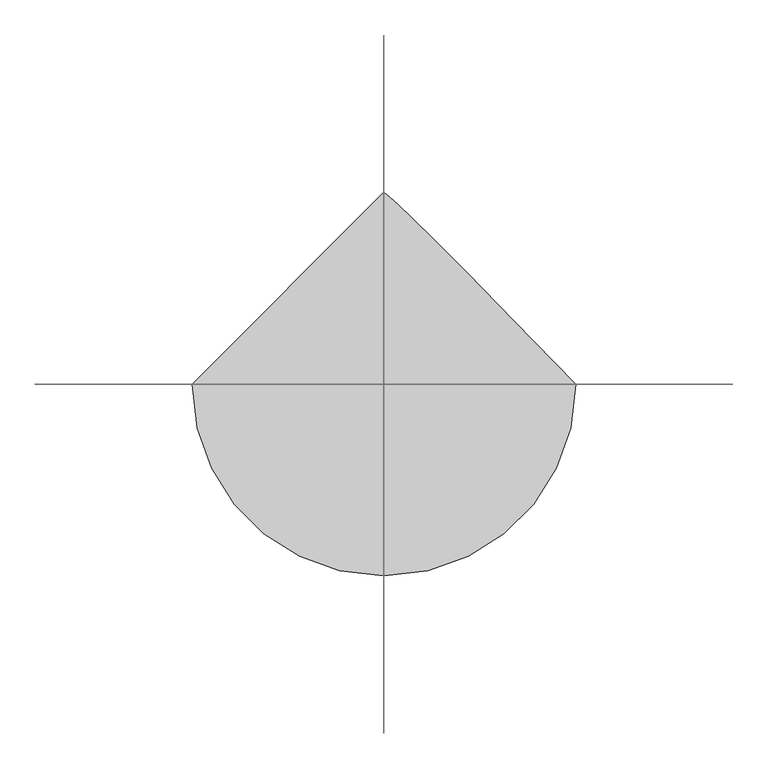
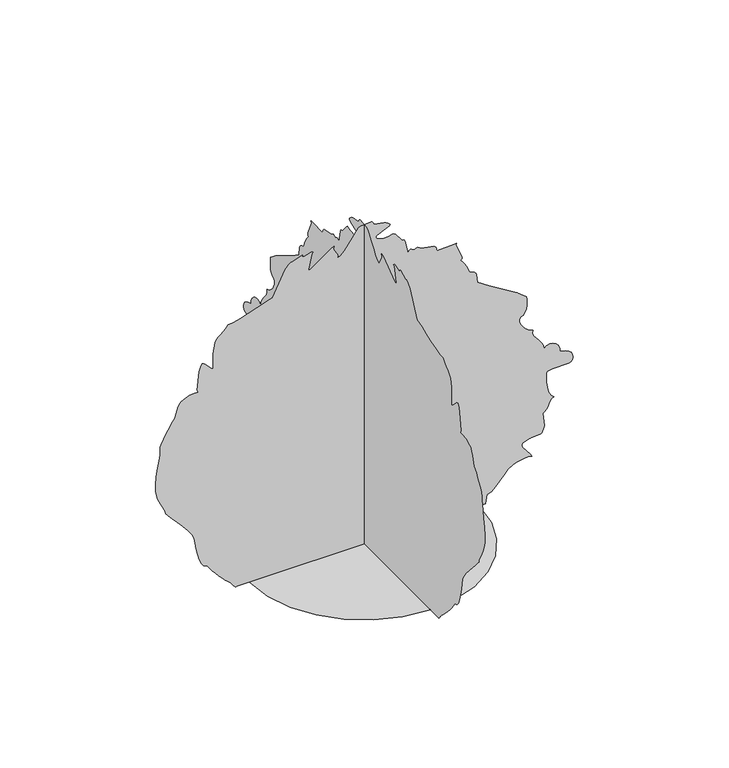
"""IFC4 building model written with IfcOpenShell, lengths in millimetres: proxy geometry, vibernum 26767 : vibernum 26767."""

import ifcopenshell
import ifcopenshell.guid

model = None  # the IFC model being written
_history = None  # IfcOwnerHistory: only IFC2X3 demands one
_inside = {}  # id of a spatial element -> (the spatial element, [elements in it])
_under = {}  # id of a project, library or spatial element -> (it, [spatial elements below it])
_declared = {}  # id of a project -> (the project, [libraries it declares])
_typed = {}  # id of a type object -> (the type object, [elements of that type])
_made_of = {}  # id of a material, layer set ... -> (it, [elements and type objects made of it])


def new_model(schema):
    """Start an empty IFC model of exactly this schema.

    Asked for "IFC4X3", IfcOpenShell would pick the latest addendum, in which some entities
    have other attributes; the version numbers below select the first issue.
    IFC2X3 requires an IfcOwnerHistory on every rooted entity: one is made here for all.
    """
    global model, _history
    if schema == "IFC4X3":
        model = ifcopenshell.file(schema_version=(4, 3, 0, 0))
    else:
        model = ifcopenshell.file(schema=schema)
    _inside.clear()
    _under.clear()
    _declared.clear()
    _typed.clear()
    _made_of.clear()
    _history = None
    if model.schema == "IFC2X3":
        org = make("IfcOrganization", Name="unknown")
        user = make(
            "IfcPersonAndOrganization",
            ThePerson=make("IfcPerson", FamilyName="unknown"),
            TheOrganization=org,
        )
        app = make(
            "IfcApplication",
            ApplicationDeveloper=org,
            Version="unknown",
            ApplicationFullName="unknown",
            ApplicationIdentifier="unknown",
        )
        _history = make(
            "IfcOwnerHistory",
            OwningUser=user,
            OwningApplication=app,
            ChangeAction="ADDED",
            CreationDate=0,
        )
    return model


def make(cls, **values):
    """One entity of the class cls with the attributes given. An attribute that is None is left unset."""
    return model.create_entity(
        cls, **{name: value for name, value in values.items() if value is not None}
    )


def rooted(cls, **values):
    """An entity with a GlobalId (a new one), such as an element, a storey or a relation."""
    return make(cls, GlobalId=ifcopenshell.guid.new(), OwnerHistory=_history, **values)


def si_unit(unit_type, name, prefix=None):
    """IfcSIUnit, for example si_unit("LENGTHUNIT", "METRE", prefix="MILLI")."""
    return make("IfcSIUnit", UnitType=unit_type, Prefix=prefix, Name=name)


def assignment(units):
    """IfcUnitAssignment: the units of a project."""
    return None if units is None else make("IfcUnitAssignment", Units=units)


def point(xyz):
    """IfcCartesianPoint."""
    return None if xyz is None else make("IfcCartesianPoint", Coordinates=xyz)


def direction(xyz):
    """IfcDirection."""
    return None if xyz is None else make("IfcDirection", DirectionRatios=xyz)


def frame(location, z_axis=None, x_axis=None):
    """IfcAxis2Placement3D, a coordinate frame: its origin and axes. An axis left out is left unset."""
    return make(
        "IfcAxis2Placement3D",
        Location=point(location),
        Axis=direction(z_axis),
        RefDirection=direction(x_axis),
    )


def origin():
    """The frame at (0, 0, 0) with its axes left unset."""
    return frame((0.0, 0.0, 0.0))


def place(relative_to, where):
    """IfcLocalPlacement: puts the frame where relative to a parent placement (None: the world)."""
    return make(
        "IfcLocalPlacement", PlacementRelTo=relative_to, RelativePlacement=where
    )


def context(
    kind, dimensions, precision=None, world=None, true_north=None, identifier=None
):
    """IfcGeometricRepresentationContext, for example the 3D "Model" context."""
    return make(
        "IfcGeometricRepresentationContext",
        ContextIdentifier=identifier,
        ContextType=kind,
        CoordinateSpaceDimension=dimensions,
        Precision=precision,
        WorldCoordinateSystem=world,
        TrueNorth=true_north,
    )


def project(units=None, contexts=None):
    """IfcProject with its units and contexts."""
    return rooted(
        "IfcProject",
        Name="project",
        RepresentationContexts=contexts,
        UnitsInContext=assignment(units),
    )


def spatial(cls, under=None, at=None, **own):
    """A site, building, storey or space (cls), placed at a placement, below another one or the project."""
    s = rooted(cls, ObjectPlacement=at, **own)
    if under is not None:
        _under.setdefault(under.id(), (under, []))[1].append(s)
    return s


def point_list(points):
    """IfcCartesianPointList2D or 3D."""
    cls = (
        "IfcCartesianPointList2D" if len(points[0]) == 2 else "IfcCartesianPointList3D"
    )
    return make(cls, CoordList=points)


def triangles(points, corners, closed=None, point_numbers=None):
    """IfcTriangulatedFaceSet: each triangle names its three corners, points numbered from 1."""
    return make(
        "IfcTriangulatedFaceSet",
        Coordinates=point_list(points),
        Closed=closed,
        CoordIndex=corners,
        PnIndex=point_numbers,
    )


def shape(context_of_items, identifier, shape_type, items):
    """IfcShapeRepresentation: the items that make up one representation, for example the "Body"."""
    return make(
        "IfcShapeRepresentation",
        ContextOfItems=context_of_items,
        RepresentationIdentifier=identifier,
        RepresentationType=shape_type,
        Items=items,
    )


def source(mapping_origin, context_of_items, identifier, shape_type, items):
    """IfcRepresentationMap: a shape defined once, which mapped items show again and again."""
    return make(
        "IfcRepresentationMap",
        MappingOrigin=mapping_origin,
        MappedRepresentation=shape(context_of_items, identifier, shape_type, items),
    )


def transform(
    local_origin,
    x_axis=None,
    y_axis=None,
    z_axis=None,
    scale=None,
    scale2=None,
    scale3=None,
    uniform=True,
):
    """IfcCartesianTransformationOperator3D, or its non-uniform kind. x_axis, y_axis, z_axis: its Axis1, 2, 3."""
    if uniform:
        return make(
            "IfcCartesianTransformationOperator3D",
            Axis1=direction(x_axis),
            Axis2=direction(y_axis),
            LocalOrigin=point(local_origin),
            Scale=scale,
            Axis3=direction(z_axis),
        )
    return make(
        "IfcCartesianTransformationOperator3DnonUniform",
        Axis1=direction(x_axis),
        Axis2=direction(y_axis),
        LocalOrigin=point(local_origin),
        Scale=scale,
        Axis3=direction(z_axis),
        Scale2=scale2,
        Scale3=scale3,
    )


def mapped(mapping_source, mapping_target):
    """IfcMappedItem: shows the shape of a source again, moved by a transform."""
    return make(
        "IfcMappedItem", MappingSource=mapping_source, MappingTarget=mapping_target
    )


def made_of(thing, what):
    """Note that an element or type object is made of a material, layer set ...; save() writes the relation."""
    if what is not None:
        _made_of.setdefault(what.id(), (what, []))[1].append(thing)
    return thing


def element(
    cls,
    number,
    at=None,
    inside=None,
    cuts=None,
    type_object=None,
    material=None,
    context=None,
    identifier="Body",
    shape_type=None,
    held_by="IfcProductDefinitionShape",
    body=None,
    shapes=None,
    **own,
):
    """One element of the class cls, such as IfcWall. Its Tag is "e" and its number.

    at: its placement. inside: the storey or other place that contains it. cuts: it is an
    opening in that element (IfcRelVoidsElement). A single representation is given by context,
    identifier, shape_type and body (its items); several are given by shapes. held_by: the class
    of the entity that holds the representations. save() writes the other relations.
    """
    e = rooted(cls, Tag="e%d" % number, ObjectPlacement=at, **own)
    if body is not None:
        shapes = [shape(context, identifier, shape_type, body)]
    if shapes is not None:
        e.Representation = make(held_by, Representations=shapes)
    if inside is not None:
        _inside.setdefault(inside.id(), (inside, []))[1].append(e)
    if cuts is not None:
        rooted(
            "IfcRelVoidsElement", RelatingBuildingElement=cuts, RelatedOpeningElement=e
        )
    if type_object is not None:
        _typed.setdefault(type_object.id(), (type_object, []))[1].append(e)
    return made_of(e, material)


def aggregate(whole, parts):
    """IfcRelAggregates: a whole, such as a stair, and the parts it consists of."""
    return rooted("IfcRelAggregates", RelatingObject=whole, RelatedObjects=parts)


def save(model, path):
    """Write the relations noted so far, then the file.

    IfcRelAggregates (storeys below a building ...), IfcRelContainedInSpatialStructure (elements
    in a storey), IfcRelDefinesByType, IfcRelAssociatesMaterial and IfcRelDeclares: one each for
    every whole, place, type object, material and project.
    """
    for whole, parts in _under.values():
        aggregate(whole, parts)
    for where, things in _inside.values():
        rooted(
            "IfcRelContainedInSpatialStructure",
            RelatedElements=things,
            RelatingStructure=where,
        )
    for kind, things in _typed.values():
        rooted("IfcRelDefinesByType", RelatedObjects=things, RelatingType=kind)
    for what, things in _made_of.values():
        rooted("IfcRelAssociatesMaterial", RelatedObjects=things, RelatingMaterial=what)
    for by, libraries in _declared.values():
        rooted("IfcRelDeclares", RelatingContext=by, RelatedDefinitions=libraries)
    model.write(path)


def entourage_5c4a15e9(model_context):
    return source(origin(), model_context, "Body", "Tessellation", [
        triangles([(-310.4009663, 0.0, 0.0), (-302.1967432, -71.1236111, 0.0), (-278.8261857, -136.4392555, 0.0), (-242.1615087, -194.0757083, 0.0), (-194.0757083, -242.1615087, 0.0), (-136.4392555, -278.8261857, 0.0), (-71.1236111, -302.1967432, 0.0), (1.36e-05, -310.4009663, 0.0), (71.1236111, -302.1967432, 0.0), (136.4392555, -278.8261857, 0.0), (194.0757083, -242.1615087, 0.0), (242.1615087, -194.0757083, 0.0), (278.8261857, -136.4392555, 0.0), (302.1967432, -71.1236111, 0.0), (310.4009663, 2.71e-05, 0.0), (209.5283262, 103.4718092, 0.0), (134.7455816, 179.6535872, 0.0), (81.7052599, 233.0934394, 0.0), (46.0591254, 268.3410517, 0.0), (23.45852, 289.9412231, 0.0), (9.5549798, 302.4456561, 0.0), (-4.07e-05, 310.4009663, 0.0), (-352.7554667, 2.15e-05, 4.3495503), (-355.9965117, 2.13e-05, 8.4826161), (-359.0826241, 2.1e-05, 12.3234041), (-362.0188548, 2.08e-05, 15.7959676), (-364.8077834, 2.07e-05, 18.8245652), (-367.457004, 2.05e-05, 21.3332227), (-369.9665528, 2.04e-05, 23.2460988), (-375.8161594, 2.01e-05, 28.5320975), (-383.5606359, 1.96e-05, 36.3306653), (-392.4582396, 1.9e-05, 45.9079945), (-401.7775108, 1.84e-05, 56.5300297), (-410.7742001, 1.78e-05, 67.463215), (-418.7091808, 1.71e-05, 77.9737471), (-424.8483773, 1.66e-05, 87.3278091), (-434.3200376, 1.64e-05, 90.3102761), (-441.518399, 1.59e-05, 99.1873323), (-446.9133459, 1.51e-05, 112.4136326), (-450.9672046, 1.41e-05, 128.4448579), (-454.1523663, 1.31e-05, 145.7354086), (-456.9311211, 1.21e-05, 162.7404662), (-459.7733894, 1.12e-05, 177.9152122), (-465.8821009, 1.05e-05, 189.8085088), (-476.9463238, 9.6e-06, 205.0848474), (-490.9620744, 8.5e-06, 222.0754346), (-505.927767, 7.5e-06, 239.1112225), (-519.8393452, 6.6e-06, 254.5234358), (-530.6927888, 5.9e-06, 266.6443348), (-536.4840051, 5.5e-06, 273.804599), (-537.980062, 5.1e-06, 279.9056801), (-541.2769901, 4.6e-06, 287.7695352), (-545.6533945, 4.1e-06, 296.6874683), (-550.3904963, 3.6e-06, 305.9584685), (-554.7669371, 3e-06, 314.8764198), (-558.0638288, 2.6e-06, 322.7377496), (-559.5599221, 2.2e-06, 328.8413741), (-564.0633173, 1.1e-06, 346.2505222), (-564.6424607, -1e-07, 367.0963428), (-562.5393188, -1.4e-06, 389.5906094), (-558.9909525, -2.8e-06, 411.9375375), (-555.2393646, -4e-06, 432.3439227), (-552.5215799, -5e-06, 449.0164879), (-552.0770576, -5.6e-06, 460.1619922), (-551.4522048, -6.2e-06, 469.7809908), (-548.1832546, -6.8e-06, 479.8495623), (-543.0422894, -7.4e-06, 490.1772022), (-536.8090942, -8.1e-06, 500.5785295), (-530.2609838, -8.7e-06, 510.8553732), (-524.1776705, -9.2e-06, 520.822352), (-519.3338891, -9.8e-06, 530.2863819), (-514.6958364, -1.01e-05, 534.5764544), (-511.1779552, -1.05e-05, 541.7037083), (-508.3280565, -1.1e-05, 550.5352913), (-505.7042341, -1.16e-05, 559.930757), (-502.8569152, -1.21e-05, 568.7597966), (-499.3364542, -1.25e-05, 575.8870505), (-494.6984015, -1.28e-05, 580.1796301), (-488.7141738, -1.3e-05, 583.3724221), (-483.0575787, -1.32e-05, 586.1308657), (-477.4467293, -1.33e-05, 588.3914835), (-471.5996298, -1.34e-05, 590.0856388), (-465.2318499, -1.35e-05, 591.1448401), (-458.0563431, -1.35e-05, 591.5029578), (-449.7962731, -1.35e-05, 591.0940438), (-452.0898831, -1.38e-05, 597.7844058), (-446.8498687, -1.69e-05, 648.1323137), (-442.8239516, -1.75e-05, 659.7223766), (-438.0639951, -1.8e-05, 668.1551468), (-434.5155925, -1.8e-05, 667.6064884), (-430.9748566, -1.79e-05, 665.0360058), (-414.5257879, -1.68e-05, 647.428723), (-409.2578319, -1.66e-05, 644.4162615), (-408.9962199, -1.74e-05, 657.4007887), (-409.1181238, -1.79e-05, 666.2653639), (-409.3213454, -1.83e-05, 672.7017443), (-409.3035413, -1.87e-05, 678.4040852), (-408.7625133, -1.91e-05, 685.0639257), (-407.3934834, -1.96e-05, 694.3755667), (-404.8915649, -2.04e-05, 708.0306198), (-403.2913719, -2.1e-05, 717.4769182), (-399.8064829, -2.14e-05, 724.3451036), (-394.8255369, -2.17e-05, 729.6460882), (-388.7295427, -2.2e-05, 734.3907841), (-381.9096102, -2.23e-05, 739.5952629), (-374.7468206, -2.27e-05, 746.2703642), (-367.6271971, -2.33e-05, 755.4296162), (-354.5182589, -2.33e-05, 756.2449734), (-335.3386883, -2.36e-05, 761.043009), (-312.9155657, -2.4e-05, 768.2718555), (-290.0885433, -2.45e-05, 776.3821163), (-269.6872632, -2.49e-05, 783.819235), (-254.5437653, -2.53e-05, 789.0313442), (-247.4939957, -2.53e-05, 790.4715179), (-213.6794536, -2.94e-05, 858.769602), (-205.2583288, -3e-05, 869.5493946), (-197.3670409, -3.03e-05, 874.0807314), (-193.2331907, -3.03e-05, 873.8495682), (-168.7295447, -3.09e-05, 884.1188541), (-166.460806, -3.09e-05, 883.4558859), (-168.0742249, -3.06e-05, 879.0896553), (-161.877383, -3.06e-05, 879.3893463), (-144.3734641, -3.09e-05, 884.8376329), (-141.0938133, -3.09e-05, 884.1543898), (-137.9627544, -3.07e-05, 881.4086271), (-140.7920603, -3.07e-05, 880.4332506), (-150.2901451, -2.82e-05, 838.0508085), (-150.4359393, -2.79e-05, 834.0097034), (-142.0369153, -2.81e-05, 837.3624784), (-89.9201382, -3.04e-05, 875.4065952), (-81.5211142, -3.06e-05, 878.7594429), (-83.236371, -3.02e-05, 872.9860308), (-82.0336828, -2.99e-05, 867.6621552), (-72.5891921, -2.9e-05, 852.5922901), (-71.3862495, -2.87e-05, 847.2684872), (-73.1015109, -2.84e-05, 841.495075), (-63.556186, -2.86e-05, 845.6047806), (-53.0855361, -2.92e-05, 856.2092932), (-42.3674857, -3.01e-05, 870.5983858), (-32.0797166, -3.1e-05, 886.0492596), (-22.9007347, -3.19e-05, 899.8541582), (-15.50783, -3.24e-05, 909.2952971), (-10.5790577, -3.25e-05, 911.6575075), (18.9106201, -3.27e-05, 914.4007267), (21.5322068, -3.27e-05, 913.1789989), (23.8564858, -3.25e-05, 909.8845779), (26.6850082, -3.21e-05, 903.8622711), (53.36646, -3.19e-05, 899.8287237), (58.7731068, -3.17e-05, 897.4639698), (63.9669031, -3.15e-05, 893.9232702), (69.0938976, -3.12e-05, 888.8939987), (68.0601171, -3.1e-05, 885.5234196), (63.3263127, -3.08e-05, 882.1706446), (34.7215748, -3.01e-05, 870.0904226), (31.9859905, -2.99e-05, 867.6900604), (32.133565, -2.97e-05, 863.7226427), (35.5686638, -2.95e-05, 860.1538925), (41.5277613, -2.93e-05, 857.2862623), (49.2473392, -2.92e-05, 855.4244574), (57.9630999, -2.92e-05, 854.8808859), (66.9122902, -2.92e-05, 855.9553116), (75.3308715, -2.94e-05, 858.9575993), (79.5358429, -2.94e-05, 858.9905914), (84.1909094, -2.92e-05, 855.1374109), (99.0570351, -2.8e-05, 835.8054514), (103.7123468, -2.78e-05, 831.9522709), (107.9173227, -2.78e-05, 831.9827196), (110.5566329, -2.75e-05, 826.9687815), (117.7400153, -2.54e-05, 791.6018269), (122.069702, -2.57e-05, 796.2169521), (125.2845857, -2.58e-05, 797.6521116), (127.9442162, -2.57e-05, 797.0729319), (133.8415943, -2.56e-05, 794.512623), (138.1999856, -2.56e-05, 794.8580961), (144.2457012, -2.58e-05, 797.8374928), (154.0983702, -2.54e-05, 791.6500797), (188.4892397, -2.5e-05, 784.7844378), (193.5639118, -2.47e-05, 779.5723286), (196.3218285, -2.41e-05, 769.7729994), (243.3426139, -2.42e-05, 771.0379658), (249.3334547, -2.43e-05, 772.2673239), (247.7520468, -2.39e-05, 766.8596598), (263.6852313, -2.17e-05, 729.0644377), (264.3888039, -2.13e-05, 722.3968941), (260.2486133, -2.11e-05, 719.5673429), (264.4396183, -2.09e-05, 715.6404751), (268.5899827, -2.05e-05, 710.080422), (272.58794, -2.02e-05, 703.4306826), (276.3268288, -1.97e-05, 696.2399878), (279.6948645, -1.93e-05, 689.0492203), (282.5828423, -1.89e-05, 682.4020243), (284.8815392, -1.86e-05, 676.8470581), (292.1535699, -1.84e-05, 674.5203833), (297.5205933, -1.82e-05, 671.6629269), (301.2772681, -1.8e-05, 668.0231054), (303.7181983, -1.78e-05, 663.3520243), (306.0880391, -1.64e-05, 640.6748474), (337.5484735, -1.51e-05, 619.285528), (412.8366832, -1.23e-05, 572.7882208), (438.1198783, -1.12e-05, 553.4791523), (439.8826341, -1.08e-05, 546.9589471), (439.9893136, -9.7e-06, 528.3128105), (438.1224217, -9.1e-06, 518.4956772), (434.833124, -8.6e-06, 509.8850836), (430.0172479, -8.2e-06, 503.634157), (423.57073, -8.1e-06, 500.8960247), (419.6083265, -7.7e-06, 495.2673712), (419.9613936, -7.3e-06, 487.2053996), (423.7561475, -6.7e-06, 477.8835849), (430.1112465, -6.1e-06, 468.4703513), (438.1503633, -5.6e-06, 460.136594), (446.9946273, -5.3e-06, 454.0533171), (455.7652765, -5.1e-06, 451.3913793), (454.5663671, -4.6e-06, 443.4767461), (457.9420332, -4.1e-06, 435.1353584), (464.2260246, -3.6e-06, 426.3952306), (471.7495116, -3.1e-06, 417.2791446), (478.8462805, -2.5e-06, 407.8151147), (483.8449943, -1.9e-06, 398.025923), (485.0794393, -1.3e-06, 387.9344968), (492.6181506, -1.7e-06, 394.3632468), (501.3405107, -1.8e-06, 396.5095548), (510.2914905, -1.8e-06, 394.9982735), (518.5109379, -1.5e-06, 390.4541831), (525.0463675, -1.1e-06, 383.5047526), (528.9401705, -5e-07, 374.7773057), (529.2322675, 0.0, 364.8966951), (543.28359, 2e-07, 361.6200783), (553.2505325, 5e-07, 356.9591709), (559.7300789, 8e-07, 351.3864369), (563.3267344, 1.2e-06, 345.3742312), (564.6424607, 1.5e-06, 339.3975975), (564.2741693, 1.9e-06, 333.9264562), (562.8263652, 2.1e-06, 329.438249), (558.5058077, 2.4e-06, 325.0237292), (551.6808246, 2.5e-06, 323.3371679), (508.3052018, 2.5e-06, 323.4667022), (495.6814084, 2.7e-06, 320.1113837), (493.0550426, 3e-06, 315.2853702), (491.9247336, 3.6e-06, 304.683401), (492.3870237, 4.5e-06, 290.5000371), (494.5434691, 5.4e-06, 274.934908), (498.4855614, 6.3e-06, 260.1850997), (504.3148567, 7e-06, 248.4462268), (512.1304407, 7.4e-06, 241.918682), (506.1944658, 7.6e-06, 237.9293542), (502.0110729, 7.9e-06, 232.375896), (498.8894248, 8.3e-06, 225.9143899), (496.1360682, 8.7e-06, 219.2011551), (493.06518, 9.1e-06, 212.8918018), (488.9859595, 9.4e-06, 207.6423766), (483.2074605, 9.6e-06, 204.1089804), (486.5094392, 1.18e-05, 167.9235982), (484.7949363, 1.23e-05, 159.1671923), (479.7174846, 1.29e-05, 149.4257811), (478.0410971, 1.3e-05, 147.3986065), (448.2189348, 1.31e-05, 145.3638107), (427.0784738, 1.35e-05, 138.6241693), (425.673872, 1.39e-05, 132.82763), (427.5890167, 1.42e-05, 126.7778539), (449.1968184, 1.58e-05, 99.5421708), (453.2709884, 1.63e-05, 91.8492719), (446.9844898, 1.62e-05, 94.1108889), (432.729982, 1.62e-05, 94.2706539), (416.3113984, 1.64e-05, 90.1472137), (414.6045259, 1.65e-05, 89.3547294), (401.3177642, 1.66e-05, 85.9130245), (388.9555827, 1.72e-05, 76.9775597), (377.2588766, 1.79e-05, 64.7009653), (365.9660339, 1.87e-05, 51.235649), (354.8103559, 1.95e-05, 38.7350312), (343.5327375, 2e-05, 29.3512471), (331.8716034, 2.03e-05, 25.2371292), (326.9541347, 2.18e-05, 4e-05), (-349.3544025, 2.18e-05, 4e-05), (-4.6e-06, -352.7554667, 4.3495758), (-4.6e-06, -355.9965117, 8.4826416), (-4.6e-06, -359.0826241, 12.3234041), (-4.6e-06, -362.0188548, 15.7959937), (-4.6e-06, -364.8077834, 18.8245902), (-4.6e-06, -367.457004, 21.3332477), (-4.6e-06, -369.9665528, 23.2460988), (-4.6e-06, -375.8161594, 28.5320975), (-4.6e-06, -383.5606359, 36.3306653), (-4.6e-06, -392.4582396, 45.9079945), (-4.6e-06, -401.7775108, 56.5300297), (-4.6e-06, -410.7742001, 67.4634693), (-4.6e-06, -418.7091808, 77.9737471), (-4.6e-06, -424.8483773, 87.3278091), (-4.6e-06, -434.3200376, 90.3102761), (-4.6e-06, -441.518399, 99.1873323), (-4.6e-06, -446.9133459, 112.4138869), (-4.6e-06, -450.9672046, 128.4448579), (-4.6e-06, -454.1523663, 145.7354086), (-4.6e-06, -456.9311211, 162.7404662), (-4.6e-06, -459.7733894, 177.9152122), (-4.6e-06, -465.8821009, 189.8085088), (-4.6e-06, -476.9463238, 205.0848474), (-4.6e-06, -490.9620744, 222.0754346), (-4.6e-06, -505.927767, 239.1112225), (-4.6e-06, -519.8393452, 254.5234358), (-4.6e-06, -530.6927888, 266.6443348), (-4.6e-06, -536.4840051, 273.804599), (-4.6e-06, -537.980062, 279.9056801), (-4.6e-06, -541.2769901, 287.7695352), (-4.6e-06, -545.6533945, 296.6874683), (-4.6e-06, -550.3904963, 305.9584685), (-4.6e-06, -554.7669371, 314.8764198), (-4.6e-06, -558.0638288, 322.7377496), (-4.6e-06, -559.5599221, 328.8413741), (-4.6e-06, -564.0633173, 346.2505222), (-4.6e-06, -564.6424607, 367.0963428), (-4.6e-06, -562.5393188, 389.5906094), (-4.6e-06, -558.9909525, 411.9375375), (-4.6e-06, -555.2393646, 432.3439227), (-4.6e-06, -552.5215799, 449.0164879), (-4.6e-06, -552.0770576, 460.1619922), (-4.6e-06, -551.4522048, 469.7809908), (-4.6e-06, -548.1832546, 479.8495623), (-4.6e-06, -543.0422894, 490.1772022), (-4.6e-06, -536.8090942, 500.5785295), (-4.6e-06, -530.2609838, 510.8553732), (-4.6e-06, -524.1776705, 520.822352), (-4.6e-06, -519.3338891, 530.2863819), (-4.6e-06, -514.6958364, 534.5764544), (-4.6e-06, -511.1779552, 541.7037083), (-4.6e-06, -508.3280565, 550.5352913), (-4.6e-06, -505.7042341, 559.930757), (-4.6e-06, -502.8569152, 568.7597966), (-4.6e-06, -499.3364542, 575.889594), (-4.6e-06, -494.6984015, 580.1796301), (-4.6e-06, -488.7141738, 583.3724221), (-4.6e-06, -483.0575787, 586.1308657), (-4.6e-06, -477.4467293, 588.3914835), (-4.6e-06, -471.5996298, 590.0856388), (-4.6e-06, -465.2318499, 591.1448401), (-4.6e-06, -458.0563431, 591.5029578), (-4.6e-06, -449.7962731, 591.0940438), (-4.6e-06, -452.0898831, 597.7844058), (-4.6e-06, -446.8498687, 648.1323137), (-4.6e-06, -442.8239516, 659.7223766), (-4.6e-06, -438.0639951, 668.1551468), (-4.6e-06, -434.5155925, 667.6064884), (-4.6e-06, -430.9748566, 665.0360058), (-4.6e-06, -414.5257879, 647.428723), (-4.6e-06, -409.2578319, 644.4162615), (-4.6e-06, -408.9962199, 657.4007887), (-4.6e-06, -409.1181238, 666.2653639), (-4.6e-06, -409.3213454, 672.7017443), (-4.6e-06, -409.3035413, 678.4040852), (-4.6e-06, -408.7625133, 685.0639257), (-4.6e-06, -407.3934834, 694.3755667), (-4.6e-06, -404.8915649, 708.0306198), (-4.6e-06, -403.2913719, 717.4769182), (-4.6e-06, -399.8064829, 724.3451036), (-4.6e-06, -394.8255369, 729.6460882), (-4.6e-06, -388.7295427, 734.3907841), (-4.6e-06, -381.9096102, 739.5952629), (-4.6e-06, -374.7468206, 746.2703642), (-4.6e-06, -367.6271971, 755.4296162), (-4.6e-06, -354.5182589, 756.2449734), (-4.6e-06, -335.3386883, 761.043009), (-4.6e-06, -312.9155657, 768.2718555), (-4.6e-06, -290.0885433, 776.3821163), (-4.6e-06, -269.6872632, 783.819235), (-4.6e-06, -254.5437653, 789.0313442), (-4.6e-06, -247.4939957, 790.4715179), (-4.6e-06, -213.6794536, 858.769602), (-4.6e-06, -205.2583288, 869.5493946), (-4.6e-06, -197.3670409, 874.0807314), (-4.6e-06, -193.2331907, 873.8495682), (-4.6e-06, -168.7295447, 884.1188541), (-4.6e-06, -166.4605516, 883.4558859), (-4.6e-06, -168.0742249, 879.0896553), (-4.6e-06, -161.877383, 879.3893463), (-4.6e-06, -144.3734641, 884.8376329), (-4.6e-06, -141.0938133, 884.1543898), (-4.6e-06, -137.9627544, 881.4086271), (-4.6e-06, -140.7920603, 880.4332506), (-4.6e-06, -150.2901451, 838.0508085), (-4.6e-06, -150.4359393, 834.0121742), (-4.6e-06, -142.0369153, 837.3624784), (-4.6e-06, -89.9201382, 875.4065952), (-4.6e-06, -81.5211142, 878.7594429), (-4.6e-06, -83.236371, 872.9860308), (-4.6e-06, -82.0336828, 867.6621552), (-4.6e-06, -72.5891921, 852.5922901), (-4.6e-06, -71.3862495, 847.2684872), (-4.6e-06, -73.1015109, 841.495075), (-4.6e-06, -63.556186, 845.6047806), (-4.6e-06, -53.0855361, 856.2092932), (-4.6e-06, -42.3674857, 870.5983858), (-4.6e-06, -32.0797166, 886.0492596), (-4.6e-06, -22.9007347, 899.8541582), (-4.6e-06, -15.50783, 909.2952971), (-4.6e-06, -10.5790577, 911.6575075), (-4.6e-06, 18.9106201, 914.4007267), (-4.6e-06, 21.5322068, 913.1789989), (-4.6e-06, 23.8564858, 909.8845779), (-4.6e-06, 26.6850082, 903.8622711), (-4.6e-06, 53.36646, 899.8287237), (-4.6e-06, 58.7731068, 897.4639698), (-4.6e-06, 63.9669031, 893.9232702), (-4.6e-06, 69.0938976, 888.8939987), (-4.6e-06, 68.0601171, 885.5234196), (-4.6e-06, 63.3263127, 882.173188), (-4.6e-06, 34.7215748, 870.0904226), (-4.6e-06, 31.9859905, 867.6900604), (-4.6e-06, 32.133565, 863.7226427), (-4.6e-06, 35.5686638, 860.1538925), (-4.6e-06, 41.5277613, 857.2862623), (-4.6e-06, 49.2473392, 855.4269281), (-4.6e-06, 57.9630999, 854.8808859), (-4.6e-06, 66.9122902, 855.9553116), (-4.6e-06, 75.3308715, 858.9575993), (-4.6e-06, 79.5358429, 858.9905914), (-4.6e-06, 84.1909094, 855.1374109), (-4.6e-06, 99.0570351, 835.8054514), (-4.6e-06, 103.7123468, 831.9522709), (-4.6e-06, 107.9173227, 831.9852631), (-4.6e-06, 110.5566329, 826.9687815), (-4.6e-06, 117.7400153, 791.6018269), (-4.6e-06, 122.069702, 796.2169521), (-4.6e-06, 125.2845857, 797.6521116), (-4.6e-06, 127.9442162, 797.0729319), (-4.6e-06, 133.8415943, 794.512623), (-4.6e-06, 138.1999856, 794.8580961), (-4.6e-06, 144.2457012, 797.8374928), (-4.6e-06, 154.0983702, 791.6500797), (-4.6e-06, 188.4892397, 784.7844378), (-4.6e-06, 193.5639118, 779.5723286), (-4.6e-06, 196.3218285, 769.7729994), (-4.6e-06, 243.3426139, 771.0379658), (-4.6e-06, 249.3334547, 772.2673239), (-4.6e-06, 247.7520468, 766.8596598), (-4.6e-06, 263.6852313, 729.0644377), (-4.6e-06, 264.3888039, 722.3968941), (-4.6e-06, 260.2486133, 719.5673429), (-4.6e-06, 264.4396183, 715.6404751), (-4.6e-06, 268.5899827, 710.080422), (-4.6e-06, 272.58794, 703.4306826), (-4.6e-06, 276.3268288, 696.2399878), (-4.6e-06, 279.6948645, 689.0492203), (-4.6e-06, 282.5828423, 682.4020243), (-4.6e-06, 284.8815392, 676.8470581), (-4.6e-06, 292.1535699, 674.5203833), (-4.6e-06, 297.5205933, 671.6629269), (-4.6e-06, 301.2772681, 668.0231054), (-4.6e-06, 303.7181983, 663.3520243), (-4.6e-06, 306.0880391, 640.6748474), (-4.6e-06, 337.5484735, 619.285528), (-4.6e-06, 412.8366832, 572.7907642), (-4.6e-06, 438.1198783, 553.4791523), (-4.6e-06, 439.8826341, 546.9589471), (-4.6e-06, 439.9893136, 528.3128105), (-4.6e-06, 438.1224217, 518.4956772), (-4.6e-06, 434.833124, 509.8850836), (-4.6e-06, 430.0172479, 503.634157), (-4.6e-06, 423.57073, 500.8960247), (-4.6e-06, 419.6083265, 495.2673712), (-4.6e-06, 419.9613936, 487.2053996), (-4.6e-06, 423.7561475, 477.8835849), (-4.6e-06, 430.1112465, 468.4703513), (-4.6e-06, 438.1503633, 460.136594), (-4.6e-06, 446.9946273, 454.0533171), (-4.6e-06, 455.7652765, 451.3913793), (-4.6e-06, 454.5663671, 443.4767461), (-4.6e-06, 457.9420332, 435.1353584), (-4.6e-06, 464.2260246, 426.3952306), (-4.6e-06, 471.7495116, 417.2791446), (-4.6e-06, 478.8462805, 407.8151147), (-4.6e-06, 483.8449943, 398.025923), (-4.6e-06, 485.0794393, 387.9344968), (-4.6e-06, 492.6181506, 394.3632468), (-4.6e-06, 501.3405107, 396.5095548), (-4.6e-06, 510.2914905, 394.9982735), (-4.6e-06, 518.5109379, 390.4541831), (-4.6e-06, 525.0463675, 383.5047526), (-4.6e-06, 528.9401705, 374.7773057), (-4.6e-06, 529.2322675, 364.8966951), (-4.6e-06, 543.28359, 361.6200783), (-4.6e-06, 553.2505325, 356.9591709), (-4.6e-06, 559.7300789, 351.3864369), (-4.6e-06, 563.3267344, 345.3742312), (-4.6e-06, 564.6424607, 339.3975975), (-4.6e-06, 564.2741693, 333.9264562), (-4.6e-06, 562.8263652, 329.438249), (-4.6e-06, 558.5058077, 325.0237292), (-4.6e-06, 551.6808246, 323.3371679), (-4.6e-06, 508.3052018, 323.4667022), (-4.6e-06, 495.6814084, 320.1113837), (-4.6e-06, 493.0550426, 315.2853702), (-4.6e-06, 491.9247336, 304.683401), (-4.6e-06, 492.3870237, 290.5000371), (-4.6e-06, 494.5434691, 274.934908), (-4.6e-06, 498.4855614, 260.1850997), (-4.6e-06, 504.3148567, 248.4464812), (-4.6e-06, 512.1304407, 241.918682), (-4.6e-06, 506.1944658, 237.9293542), (-4.6e-06, 502.0110729, 232.375896), (-4.6e-06, 498.8894248, 225.9143899), (-4.6e-06, 496.1360682, 219.2011551), (-4.6e-06, 493.06518, 212.8918018), (-4.6e-06, 488.9859595, 207.6423766), (-4.6e-06, 483.2074605, 204.1089804), (-4.6e-06, 486.5094392, 167.9235982), (-4.6e-06, 484.7949363, 159.1671923), (-4.6e-06, 479.7174846, 149.4257811), (-4.6e-06, 478.0410971, 147.3988609), (-4.6e-06, 448.2189348, 145.3638107), (-4.6e-06, 427.0784738, 138.6241693), (-4.6e-06, 425.673872, 132.8278843), (-4.6e-06, 427.5890167, 126.7778539), (-4.6e-06, 449.1968184, 99.5421708), (-4.6e-06, 453.2709884, 91.8492719), (-4.6e-06, 446.9844898, 94.1108889), (-4.6e-06, 432.729982, 94.2706539), (-4.6e-06, 416.3113984, 90.1472137), (-4.6e-06, 414.6045259, 89.3547294), (-4.6e-06, 401.3177642, 85.9130245), (-4.6e-06, 388.9555827, 76.9775597), (-4.6e-06, 377.2588766, 64.7009653), (-4.6e-06, 365.9660339, 51.235649), (-4.6e-06, 354.8103559, 38.7350312), (-4.6e-06, 343.5327375, 29.3512471), (-4.6e-06, 331.8716034, 25.2371564), (-4.6e-06, 326.9541347, 6.03e-05), (-4.6e-06, -349.3544025, 6.03e-05)], [[21, 22, 1], [20, 21, 1], [19, 20, 1], [18, 19, 1], [17, 18, 1], [17, 1, 2], [17, 2, 3], [17, 3, 4], [16, 17, 4], [16, 4, 5], [16, 5, 6], [16, 6, 7], [16, 7, 8], [16, 8, 9], [16, 9, 10], [16, 10, 11], [16, 11, 12], [15, 16, 12], [14, 15, 12], [13, 14, 12], [261, 262, 263], [130, 131, 132], [124, 125, 126], [180, 181, 182], [244, 245, 246], [119, 120, 121], [118, 119, 121], [212, 213, 214], [273, 274, 275], [123, 124, 126], [260, 261, 263], [88, 89, 90], [88, 90, 91], [260, 263, 264], [87, 88, 91], [87, 91, 92], [122, 123, 126], [166, 167, 168], [150, 151, 152], [150, 152, 153], [149, 150, 153], [148, 149, 153], [148, 153, 154], [147, 148, 154], [147, 154, 155], [87, 92, 93], [183, 184, 185], [122, 126, 127], [121, 122, 127], [174, 175, 176], [130, 132, 133], [129, 130, 133], [260, 264, 265], [129, 133, 134], [129, 134, 135], [129, 135, 136], [273, 275, 23], [86, 87, 93], [85, 86, 93], [273, 23, 24], [273, 24, 25], [273, 25, 26], [118, 121, 127], [118, 127, 128], [106, 107, 108], [273, 26, 27], [260, 265, 266], [260, 266, 267], [259, 260, 267], [244, 246, 247], [179, 180, 182], [273, 27, 28], [255, 256, 257], [162, 163, 164], [161, 162, 164], [117, 118, 128], [116, 117, 128], [115, 116, 128], [114, 115, 128], [273, 28, 29], [273, 29, 30], [273, 30, 31], [273, 31, 32], [273, 32, 33], [273, 33, 34], [273, 34, 35], [273, 35, 36], [161, 164, 165], [170, 171, 172], [169, 170, 172], [169, 172, 173], [254, 255, 257], [253, 254, 257], [252, 253, 257], [252, 257, 258], [243, 244, 247], [160, 161, 165], [36, 37, 38], [243, 247, 248], [36, 38, 39], [273, 36, 39], [273, 39, 40], [273, 40, 41], [273, 41, 42], [273, 42, 43], [273, 43, 44], [273, 44, 45], [273, 45, 46], [273, 46, 47], [272, 273, 47], [271, 272, 47], [270, 271, 47], [269, 270, 47], [268, 269, 47], [267, 268, 47], [259, 267, 47], [258, 259, 47], [252, 258, 47], [252, 47, 48], [252, 48, 49], [252, 49, 50], [252, 50, 51], [252, 51, 52], [252, 52, 53], [252, 53, 54], [252, 54, 55], [252, 55, 56], [252, 56, 57], [252, 57, 58], [252, 58, 59], [252, 59, 60], [252, 60, 61], [252, 61, 62], [252, 62, 63], [252, 63, 64], [252, 64, 65], [252, 65, 66], [252, 66, 67], [252, 67, 68], [252, 68, 69], [252, 69, 70], [252, 70, 71], [252, 71, 72], [252, 72, 73], [252, 73, 74], [252, 74, 75], [252, 75, 76], [252, 76, 77], [252, 77, 78], [252, 78, 79], [252, 79, 80], [252, 80, 81], [252, 81, 82], [252, 82, 83], [252, 83, 84], [252, 84, 85], [252, 85, 93], [252, 93, 94], [252, 94, 95], [252, 95, 96], [252, 96, 97], [252, 97, 98], [252, 98, 99], [252, 99, 100], [252, 100, 101], [252, 101, 102], [252, 102, 103], [252, 103, 104], [252, 104, 105], [252, 105, 106], [252, 106, 108], [252, 108, 109], [252, 109, 110], [252, 110, 111], [252, 111, 112], [252, 112, 113], [252, 113, 114], [252, 114, 128], [252, 128, 129], [252, 129, 136], [252, 136, 137], [252, 137, 138], [251, 252, 138], [250, 251, 138], [249, 250, 138], [248, 249, 138], [243, 248, 138], [242, 243, 138], [241, 242, 138], [240, 241, 138], [239, 240, 138], [238, 239, 138], [238, 138, 139], [238, 139, 140], [238, 140, 141], [238, 141, 142], [238, 142, 143], [237, 238, 143], [234, 235, 236], [233, 234, 236], [232, 233, 236], [231, 232, 236], [230, 231, 236], [229, 230, 236], [228, 229, 236], [227, 228, 236], [227, 236, 237], [179, 182, 183], [179, 183, 185], [199, 200, 201], [199, 201, 202], [199, 202, 203], [199, 203, 204], [199, 204, 205], [199, 205, 206], [199, 206, 207], [198, 199, 207], [198, 207, 208], [144, 145, 146], [144, 146, 147], [144, 147, 155], [143, 144, 155], [143, 155, 156], [237, 143, 156], [237, 156, 157], [237, 157, 158], [237, 158, 159], [237, 159, 160], [177, 178, 179], [226, 227, 237], [225, 226, 237], [224, 225, 237], [223, 224, 237], [222, 223, 237], [221, 222, 237], [220, 221, 237], [220, 237, 160], [219, 220, 160], [218, 219, 160], [166, 168, 169], [165, 166, 169], [160, 165, 169], [218, 160, 169], [217, 218, 169], [216, 217, 169], [215, 216, 169], [215, 169, 173], [215, 173, 174], [215, 174, 176], [211, 212, 214], [211, 214, 215], [194, 195, 196], [193, 194, 196], [192, 193, 196], [192, 196, 197], [197, 198, 208], [176, 177, 179], [197, 208, 209], [176, 179, 185], [185, 186, 187], [176, 185, 187], [176, 187, 188], [176, 188, 189], [176, 189, 190], [176, 190, 191], [176, 191, 192], [176, 192, 197], [176, 197, 209], [176, 209, 210], [215, 176, 210], [211, 215, 210], [514, 515, 516], [383, 384, 385], [377, 378, 379], [433, 434, 435], [497, 498, 499], [372, 373, 374], [371, 372, 374], [465, 466, 467], [526, 527, 528], [376, 377, 379], [513, 514, 516], [341, 342, 343], [341, 343, 344], [513, 516, 517], [340, 341, 344], [340, 344, 345], [375, 376, 379], [419, 420, 421], [403, 404, 405], [403, 405, 406], [402, 403, 406], [401, 402, 406], [401, 406, 407], [400, 401, 407], [400, 407, 408], [340, 345, 346], [436, 437, 438], [375, 379, 380], [374, 375, 380], [427, 428, 429], [383, 385, 386], [382, 383, 386], [513, 517, 518], [382, 386, 387], [382, 387, 388], [382, 388, 389], [526, 528, 276], [339, 340, 346], [338, 339, 346], [526, 276, 277], [526, 277, 278], [526, 278, 279], [371, 374, 380], [371, 380, 381], [359, 360, 361], [526, 279, 280], [513, 518, 519], [513, 519, 520], [512, 513, 520], [497, 499, 500], [432, 433, 435], [526, 280, 281], [508, 509, 510], [415, 416, 417], [414, 415, 417], [370, 371, 381], [369, 370, 381], [368, 369, 381], [367, 368, 381], [526, 281, 282], [526, 282, 283], [526, 283, 284], [526, 284, 285], [526, 285, 286], [526, 286, 287], [526, 287, 288], [526, 288, 289], [414, 417, 418], [423, 424, 425], [422, 423, 425], [422, 425, 426], [507, 508, 510], [506, 507, 510], [505, 506, 510], [505, 510, 511], [496, 497, 500], [413, 414, 418], [289, 290, 291], [496, 500, 501], [289, 291, 292], [526, 289, 292], [526, 292, 293], [526, 293, 294], [526, 294, 295], [526, 295, 296], [526, 296, 297], [526, 297, 298], [526, 298, 299], [526, 299, 300], [525, 526, 300], [524, 525, 300], [523, 524, 300], [522, 523, 300], [521, 522, 300], [520, 521, 300], [512, 520, 300], [511, 512, 300], [505, 511, 300], [505, 300, 301], [505, 301, 302], [505, 302, 303], [505, 303, 304], [505, 304, 305], [505, 305, 306], [505, 306, 307], [505, 307, 308], [505, 308, 309], [505, 309, 310], [505, 310, 311], [505, 311, 312], [505, 312, 313], [505, 313, 314], [505, 314, 315], [505, 315, 316], [505, 316, 317], [505, 317, 318], [505, 318, 319], [505, 319, 320], [505, 320, 321], [505, 321, 322], [505, 322, 323], [505, 323, 324], [505, 324, 325], [505, 325, 326], [505, 326, 327], [505, 327, 328], [505, 328, 329], [505, 329, 330], [505, 330, 331], [505, 331, 332], [505, 332, 333], [505, 333, 334], [505, 334, 335], [505, 335, 336], [505, 336, 337], [505, 337, 338], [505, 338, 346], [505, 346, 347], [505, 347, 348], [505, 348, 349], [505, 349, 350], [505, 350, 351], [505, 351, 352], [505, 352, 353], [505, 353, 354], [505, 354, 355], [505, 355, 356], [505, 356, 357], [505, 357, 358], [505, 358, 359], [505, 359, 361], [505, 361, 362], [505, 362, 363], [505, 363, 364], [505, 364, 365], [505, 365, 366], [505, 366, 367], [505, 367, 381], [505, 381, 382], [505, 382, 389], [505, 389, 390], [505, 390, 391], [504, 505, 391], [503, 504, 391], [502, 503, 391], [501, 502, 391], [496, 501, 391], [495, 496, 391], [494, 495, 391], [493, 494, 391], [492, 493, 391], [491, 492, 391], [491, 391, 392], [491, 392, 393], [491, 393, 394], [491, 394, 395], [491, 395, 396], [490, 491, 396], [487, 488, 489], [486, 487, 489], [485, 486, 489], [484, 485, 489], [483, 484, 489], [482, 483, 489], [481, 482, 489], [480, 481, 489], [480, 489, 490], [432, 435, 436], [432, 436, 438], [452, 453, 454], [452, 454, 455], [452, 455, 456], [452, 456, 457], [452, 457, 458], [452, 458, 459], [452, 459, 460], [451, 452, 460], [451, 460, 461], [397, 398, 399], [397, 399, 400], [397, 400, 408], [396, 397, 408], [396, 408, 409], [490, 396, 409], [490, 409, 410], [490, 410, 411], [490, 411, 412], [490, 412, 413], [430, 431, 432], [479, 480, 490], [478, 479, 490], [477, 478, 490], [476, 477, 490], [475, 476, 490], [474, 475, 490], [473, 474, 490], [473, 490, 413], [472, 473, 413], [471, 472, 413], [419, 421, 422], [418, 419, 422], [413, 418, 422], [471, 413, 422], [470, 471, 422], [469, 470, 422], [468, 469, 422], [468, 422, 426], [468, 426, 427], [468, 427, 429], [464, 465, 467], [464, 467, 468], [447, 448, 449], [446, 447, 449], [445, 446, 449], [445, 449, 450], [450, 451, 461], [429, 430, 432], [450, 461, 462], [429, 432, 438], [438, 439, 440], [429, 438, 440], [429, 440, 441], [429, 441, 442], [429, 442, 443], [429, 443, 444], [429, 444, 445], [429, 445, 450], [429, 450, 462], [429, 462, 463], [468, 429, 463], [464, 468, 463]], closed=False),
    ])


if __name__ == "__main__":
    model = new_model("IFC4")
    model_context = context("Model", 3, world=origin())
    ifc_project = project(units=[si_unit("LENGTHUNIT", "METRE", prefix="MILLI")], contexts=[model_context])
    site = spatial("IfcSite", under=ifc_project)
    building = spatial("IfcBuilding", under=site)
    placement = place(None, origin())
    entourage_shape = entourage_5c4a15e9(model_context)
    element("IfcBuildingElementProxy", 1, Name="vibernum 26767 : vibernum 26767", ObjectType="vibernum 26767 : vibernum 26767", at=placement, inside=building, context=model_context, shape_type="MappedRepresentation", body=[
        mapped(entourage_shape, transform((0.0, 0.0, 0.0), x_axis=(1.0, 0.0, 0.0), y_axis=(0.0, 1.0, 0.0), z_axis=(0.0, 0.0, 1.0))),
    ])
    save(model, "model.ifc")

# Revit data of these elements
# Project information
#   Project Issue Date = "Issue Date"
#   Project Status = "Project Status"
#   Client Name = "Owner"
#   Project Address = "Enter address here"
#   Project Name = "Project Name"
#   Project Number = "Project Number"
# Type "vibernum 26767 : vibernum 26767"
#   built-in parameter 1005195 = "RPC-16-FU5P-8RFX-7Q0N-4000-ST1L-LVER-AU"
#   Height = 0
